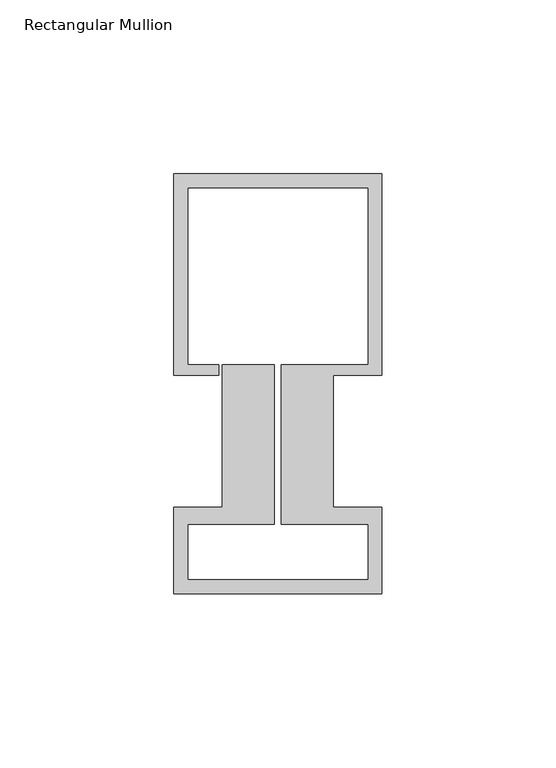
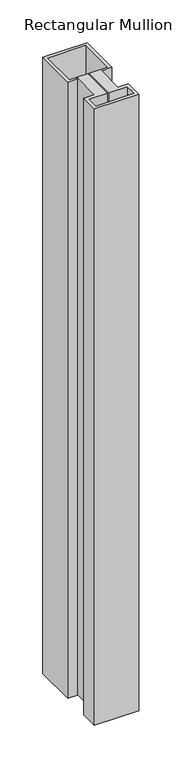
"""IFC4 building model written with IfcOpenShell, lengths in millimetres: member geometry, Rectangular Mullion : Schueco_FWS-60-SI_Tran_CovCap-20mm_Tran-55mm."""

from ifc_helpers import new_model, si_unit, frame, origin, place, context, project, spatial, polyline, outline, extrude, source, transform, mapped, element, save


def rectangular_mullion_d5ec5f76(model_context):
    return source(origin(), model_context, "Body", "SweptSolid", [
        extrude(outline(polyline([(0.0, 96.0), (0.0, 38.0), (-14.0, 38.0), (-14.0, -0.1), (0.0, -0.1), (0.0, -25.0), (-60.0, -25.0), (-60.0, -0.1), (-46.0, -0.1), (-46.0, 41.0), (-31.0, 41.0), (-31.0, -5.0), (-56.0, -5.0), (-56.0, -21.0), (-4.0, -21.0), (-4.0, -5.0), (-29.0, -5.0), (-29.0, 41.0), (-4.0, 41.0), (-4.0, 92.0), (-56.0, 92.0), (-56.0, 41.0), (-47.0, 41.0), (-47.0, 38.0), (-60.0, 38.0), (-60.0, 96.0), (0.0, 96.0)])), frame((0.0, 0.0, -880.0), z_axis=(0.0, 0.0, 1.0), x_axis=(1.0, 0.0, 0.0)), (0.0, 0.0, 1.0), 880.0),
    ])


if __name__ == "__main__":
    model = new_model("IFC4")
    model_context = context("Model", 3, world=origin())
    ifc_project = project(units=[si_unit("LENGTHUNIT", "METRE", prefix="MILLI")], contexts=[model_context])
    site = spatial("IfcSite", under=ifc_project)
    building = spatial("IfcBuilding", under=site)
    placement = place(None, origin())
    rectangular_mullion_shape = rectangular_mullion_d5ec5f76(model_context)
    element("IfcMember", 1, ObjectType="Rectangular Mullion : Schueco_FWS-60-SI_Tran_CovCap-20mm_Tran-55mm", at=placement, inside=building, context=model_context, shape_type="MappedRepresentation", body=[
        mapped(rectangular_mullion_shape, transform((0.0, 0.0, 0.0), x_axis=(1.0, 0.0, 0.0), y_axis=(0.0, 1.0, 0.0), z_axis=(0.0, 0.0, 1.0))),
    ])
    save(model, "model.ifc")

# Revit data of these elements
# Type "Rectangular Mullion : Schueco_FWS-60-SI_Tran_CovCap-20mm_Tran-55mm"
#   Model = "FWS 60.SI"
#   Manufacturer = "Schueco International KG"
#   Type Comments = "Transom"
#   Schueco thermal insulation standard = "Suitable for passive houses"
#   Burglar resistance = "RC 3"
#   Thermal insulation = "to 0.70 W/(m²K)"
#   built-in parameter 1007322 = 0.396982 (stored number, unit not read)
#   built-in parameter 1007321 = 0.0524934 (stored number, unit not read)
#   built-in parameter 1007320 = 0.0524934 (stored number, unit not read)
# Element 1 (IfcMember, "Rectangular Mullion : Schueco_FWS-60-SI_Tran_CovCap-20mm_Tran-55mm")
#   Materials on its faces: "Alu"
# Materials
#   "Alu": class "Glas", colour RGB 140 140 140, transparency 0
